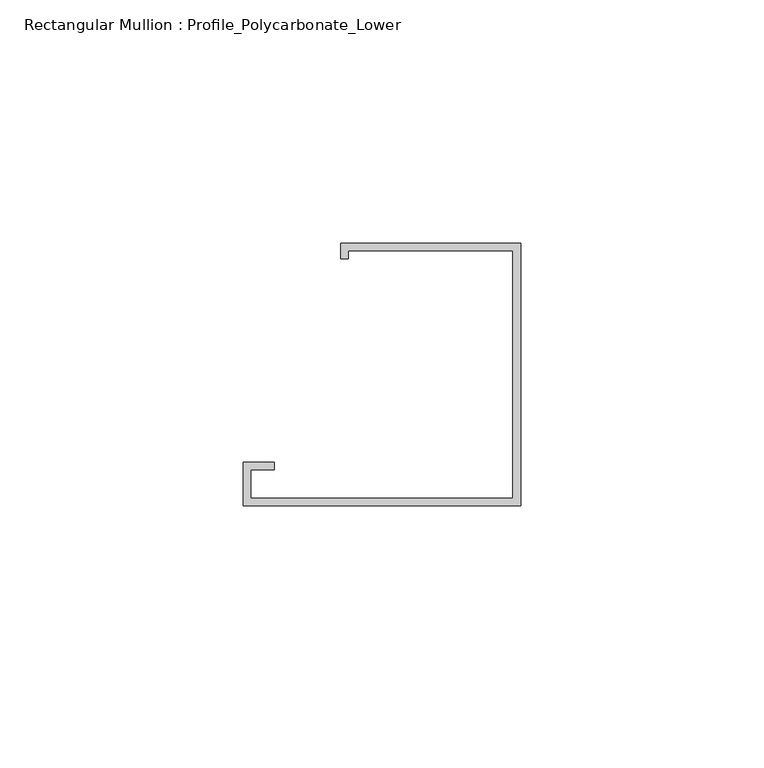
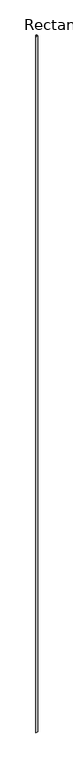
"""IFC4 building model written with IfcOpenShell, lengths in millimetres: member geometry, Rectangular Mullion : Profile_Polycarbonate_Lower."""

from ifc_helpers import new_model, si_unit, frame, origin, place, context, project, spatial, polyline, outline, extrude, source, transform, mapped, element, save


def rectangular_mullion_profile_polycarbonate_lower_d1a24a39(model_context):
    return source(origin(), model_context, "Body", "SweptSolid", [
        extrude(outline(polyline([(0.0, -28.984575), (-56.9976, -28.984575), (-56.9976, -19.992975), (-50.6476, -19.992975), (-50.6476, -21.580475), (-55.4101, -21.580475), (-55.4101, -27.397075), (-1.5875, -27.397075), (-1.5875, 23.428325), (-35.3949, 23.428325), (-35.3949, 21.840825), (-36.9824, 21.840825), (-36.9824, 25.015825), (0.0, 25.015825), (0.0, -28.984575)])), frame((0.0, 0.0, -22066.25), z_axis=(0.0, 0.0, 1.0), x_axis=(1.0, 0.0, 0.0)), (0.0, 0.0, 1.0), 22066.25),
    ])


if __name__ == "__main__":
    model = new_model("IFC4")
    model_context = context("Model", 3, world=origin())
    ifc_project = project(units=[si_unit("LENGTHUNIT", "METRE", prefix="MILLI")], contexts=[model_context])
    site = spatial("IfcSite", under=ifc_project)
    building = spatial("IfcBuilding", under=site)
    placement = place(None, origin())
    rectangular_mullion_profile_polycarbonate_lower_shape = rectangular_mullion_profile_polycarbonate_lower_d1a24a39(model_context)
    element("IfcMember", 1, ObjectType="Rectangular Mullion : Profile_Polycarbonate_Lower", at=placement, inside=building, context=model_context, shape_type="MappedRepresentation", body=[
        mapped(rectangular_mullion_profile_polycarbonate_lower_shape, transform((0.0, 0.0, 0.0), x_axis=(1.0, 0.0, 0.0), y_axis=(0.0, 1.0, 0.0), z_axis=(0.0, 0.0, 1.0))),
    ])
    save(model, "model.ifc")

# Revit data of these elements
# Type "Rectangular Mullion : Profile_Polycarbonate_Lower"
#   built-in parameter 1007322 = 0.177167 (stored number, unit not read)
#   built-in parameter 1007321 = 0 (stored number, unit not read)
#   built-in parameter 1007320 = 0.00520833 (stored number, unit not read)
